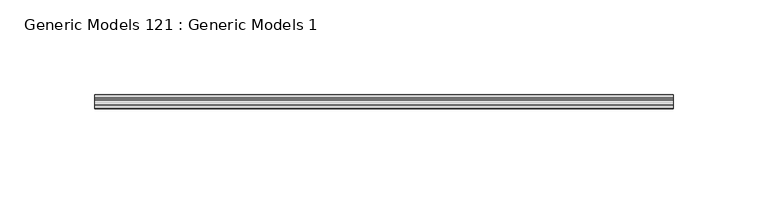
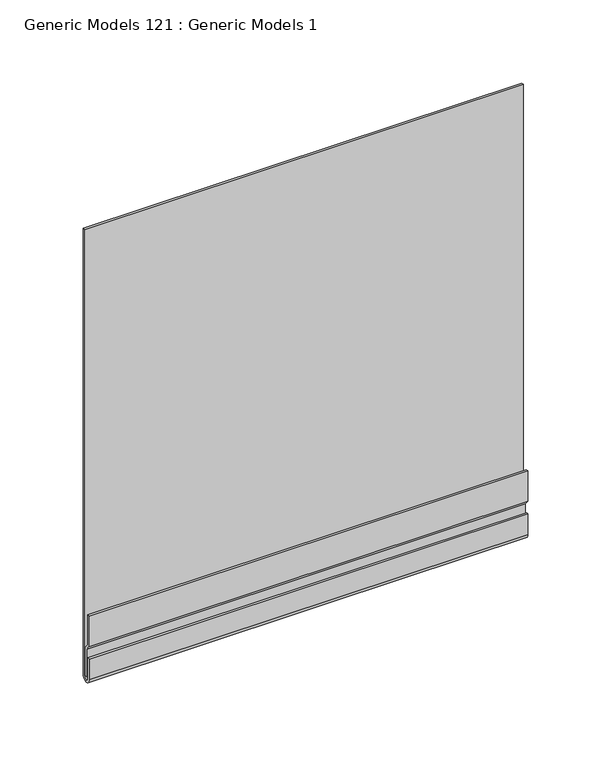
"""IFC4 building model written with IfcOpenShell, lengths in millimetres: proxy geometry, Generic Models 121 : Generic Models 1."""

from ifc_helpers import new_model, si_unit, point, frame, frame_2d, origin, place, context, project, spatial, polyline, circle_curve, trimmed, segment, composite_curve, outline, extrude, source, transform, mapped, element, save


def generic_models_121_generic_models_1_102601ae(model_context):
    return source(origin(), model_context, "Body", "SweptSolid", [
        extrude(outline(composite_curve([segment(polyline([(12629.3244905, 129249.1049552), (12629.3244905, 129264.3571776), (12630.9119905, 129264.3571776), (12630.9119905, 129249.1049552)]), True, "CONTINUOUS"), segment(trimmed(circle_curve(frame_2d((12632.9982477, 129249.1049552)), 2.0862572), [point((12630.9119905, 129249.1049552))], [point((12635.084505, 129249.1049552))], True, "CARTESIAN"), True, "CONTINUOUS"), segment(polyline([(12635.084505, 129249.1049552), (12635.084505, 129576.3330344), (12636.672005, 129576.3330344), (12636.672005, 129249.1049552)]), True, "CONTINUOUS"), segment(trimmed(circle_curve(frame_2d((12632.9982477, 129249.1049552)), 3.6737572), [point((12636.672005, 129249.1049552))], [point((12629.3244905, 129249.1049552))], False, "CARTESIAN"), True, "CONTINUOUS")], self_intersect=False)), frame((1084.7910488, 0.0, 0.0), z_axis=(1.0, 0.0, 0.0), x_axis=(0.0, 1.0, 0.0)), (0.0, 0.0, 1.0), 304.8),
        extrude(outline(polyline([(12633.9182227, 129270.4080691), (12633.9182227, 129249.6045445), (12632.3307227, 129249.6045445), (12632.3307227, 129269.8533538), (12629.5769662, 129273.3126249), (12629.5769662, 129295.7653507), (12631.1644662, 129295.7653507), (12631.1644662, 129273.8673402), (12633.9182227, 129270.4080691)])), frame((1084.7910488, 0.0, 0.0), z_axis=(1.0, 0.0, 0.0), x_axis=(0.0, 1.0, 0.0)), (0.0, 0.0, 1.0), 304.8),
    ])


if __name__ == "__main__":
    model = new_model("IFC4")
    model_context = context("Model", 3, world=origin())
    ifc_project = project(units=[si_unit("LENGTHUNIT", "METRE", prefix="MILLI")], contexts=[model_context])
    site = spatial("IfcSite", under=ifc_project)
    building = spatial("IfcBuilding", under=site)
    placement = place(None, origin())
    generic_models_121_generic_models_1_shape = generic_models_121_generic_models_1_102601ae(model_context)
    element("IfcBuildingElementProxy", 1, Name="Generic Models 121 : Generic Models 1", ObjectType="Generic Models 121 : Generic Models 1", at=placement, inside=building, context=model_context, shape_type="MappedRepresentation", body=[
        mapped(generic_models_121_generic_models_1_shape, transform((0.0, 0.0, 0.0), x_axis=(1.0, 0.0, 0.0), y_axis=(0.0, 1.0, 0.0), z_axis=(0.0, 0.0, 1.0))),
    ])
    save(model, "model.ifc")

# Revit data of these elements
# Element 1 (IfcBuildingElementProxy, "Generic Models 121 : Generic Models 1")
#   Materials on its faces: "_16 GA. COPPER BRAKE METAL FLASHING"
# Materials
#   "_16 GA. COPPER BRAKE METAL FLASHING": class "Generic", colour RGB 175 175 175, transparency 0, Cost = 0
